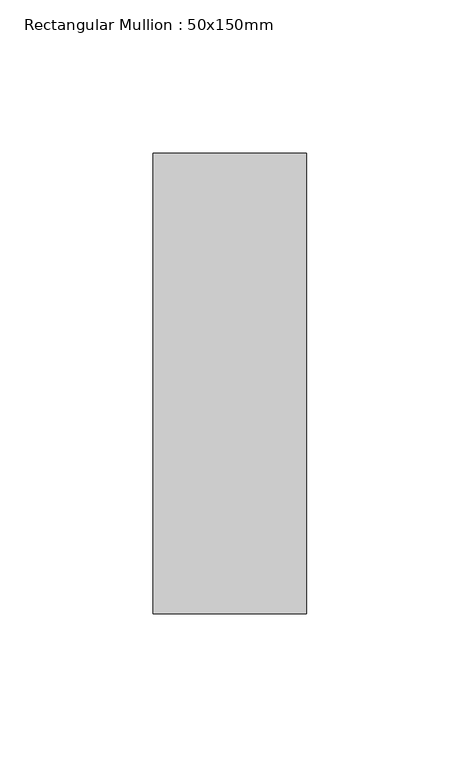
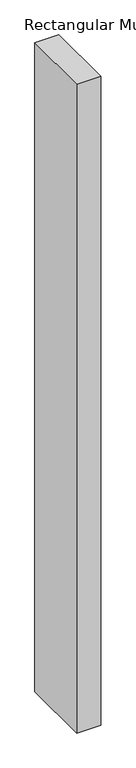
"""IFC4 building model written with IfcOpenShell, lengths in millimetres: member geometry, Rectangular Mullion : 50x150mm."""

import ifcopenshell
import ifcopenshell.guid

model = None  # the IFC model being written
_history = None  # IfcOwnerHistory: only IFC2X3 demands one
_inside = {}  # id of a spatial element -> (the spatial element, [elements in it])
_under = {}  # id of a project, library or spatial element -> (it, [spatial elements below it])
_declared = {}  # id of a project -> (the project, [libraries it declares])
_typed = {}  # id of a type object -> (the type object, [elements of that type])
_made_of = {}  # id of a material, layer set ... -> (it, [elements and type objects made of it])


def new_model(schema):
    """Start an empty IFC model of exactly this schema.

    Asked for "IFC4X3", IfcOpenShell would pick the latest addendum, in which some entities
    have other attributes; the version numbers below select the first issue.
    IFC2X3 requires an IfcOwnerHistory on every rooted entity: one is made here for all.
    """
    global model, _history
    if schema == "IFC4X3":
        model = ifcopenshell.file(schema_version=(4, 3, 0, 0))
    else:
        model = ifcopenshell.file(schema=schema)
    _inside.clear()
    _under.clear()
    _declared.clear()
    _typed.clear()
    _made_of.clear()
    _history = None
    if model.schema == "IFC2X3":
        org = make("IfcOrganization", Name="unknown")
        user = make(
            "IfcPersonAndOrganization",
            ThePerson=make("IfcPerson", FamilyName="unknown"),
            TheOrganization=org,
        )
        app = make(
            "IfcApplication",
            ApplicationDeveloper=org,
            Version="unknown",
            ApplicationFullName="unknown",
            ApplicationIdentifier="unknown",
        )
        _history = make(
            "IfcOwnerHistory",
            OwningUser=user,
            OwningApplication=app,
            ChangeAction="ADDED",
            CreationDate=0,
        )
    return model


def make(cls, **values):
    """One entity of the class cls with the attributes given. An attribute that is None is left unset."""
    return model.create_entity(
        cls, **{name: value for name, value in values.items() if value is not None}
    )


def rooted(cls, **values):
    """An entity with a GlobalId (a new one), such as an element, a storey or a relation."""
    return make(cls, GlobalId=ifcopenshell.guid.new(), OwnerHistory=_history, **values)


def si_unit(unit_type, name, prefix=None):
    """IfcSIUnit, for example si_unit("LENGTHUNIT", "METRE", prefix="MILLI")."""
    return make("IfcSIUnit", UnitType=unit_type, Prefix=prefix, Name=name)


def assignment(units):
    """IfcUnitAssignment: the units of a project."""
    return None if units is None else make("IfcUnitAssignment", Units=units)


def point(xyz):
    """IfcCartesianPoint."""
    return None if xyz is None else make("IfcCartesianPoint", Coordinates=xyz)


def direction(xyz):
    """IfcDirection."""
    return None if xyz is None else make("IfcDirection", DirectionRatios=xyz)


def frame(location, z_axis=None, x_axis=None):
    """IfcAxis2Placement3D, a coordinate frame: its origin and axes. An axis left out is left unset."""
    return make(
        "IfcAxis2Placement3D",
        Location=point(location),
        Axis=direction(z_axis),
        RefDirection=direction(x_axis),
    )


def origin():
    """The frame at (0, 0, 0) with its axes left unset."""
    return frame((0.0, 0.0, 0.0))


def place(relative_to, where):
    """IfcLocalPlacement: puts the frame where relative to a parent placement (None: the world)."""
    return make(
        "IfcLocalPlacement", PlacementRelTo=relative_to, RelativePlacement=where
    )


def context(
    kind, dimensions, precision=None, world=None, true_north=None, identifier=None
):
    """IfcGeometricRepresentationContext, for example the 3D "Model" context."""
    return make(
        "IfcGeometricRepresentationContext",
        ContextIdentifier=identifier,
        ContextType=kind,
        CoordinateSpaceDimension=dimensions,
        Precision=precision,
        WorldCoordinateSystem=world,
        TrueNorth=true_north,
    )


def project(units=None, contexts=None):
    """IfcProject with its units and contexts."""
    return rooted(
        "IfcProject",
        Name="project",
        RepresentationContexts=contexts,
        UnitsInContext=assignment(units),
    )


def spatial(cls, under=None, at=None, **own):
    """A site, building, storey or space (cls), placed at a placement, below another one or the project."""
    s = rooted(cls, ObjectPlacement=at, **own)
    if under is not None:
        _under.setdefault(under.id(), (under, []))[1].append(s)
    return s


def polyline(points):
    """IfcPolyline through the points."""
    return make("IfcPolyline", Points=[point(p) for p in points])


def outline(outer, holes=None, kind="AREA"):
    """IfcArbitraryClosedProfileDef: a profile drawn as a closed curve; with holes, ...WithVoids."""
    if holes is None:
        return make("IfcArbitraryClosedProfileDef", ProfileType=kind, OuterCurve=outer)
    return make(
        "IfcArbitraryProfileDefWithVoids",
        ProfileType=kind,
        OuterCurve=outer,
        InnerCurves=holes,
    )


def extrude(swept, where, along, depth):
    """IfcExtrudedAreaSolid: the profile swept, set in the frame where, extruded along a direction by depth."""
    return make(
        "IfcExtrudedAreaSolid",
        SweptArea=swept,
        Position=where,
        ExtrudedDirection=direction(along),
        Depth=depth,
    )


def shape(context_of_items, identifier, shape_type, items):
    """IfcShapeRepresentation: the items that make up one representation, for example the "Body"."""
    return make(
        "IfcShapeRepresentation",
        ContextOfItems=context_of_items,
        RepresentationIdentifier=identifier,
        RepresentationType=shape_type,
        Items=items,
    )


def source(mapping_origin, context_of_items, identifier, shape_type, items):
    """IfcRepresentationMap: a shape defined once, which mapped items show again and again."""
    return make(
        "IfcRepresentationMap",
        MappingOrigin=mapping_origin,
        MappedRepresentation=shape(context_of_items, identifier, shape_type, items),
    )


def transform(
    local_origin,
    x_axis=None,
    y_axis=None,
    z_axis=None,
    scale=None,
    scale2=None,
    scale3=None,
    uniform=True,
):
    """IfcCartesianTransformationOperator3D, or its non-uniform kind. x_axis, y_axis, z_axis: its Axis1, 2, 3."""
    if uniform:
        return make(
            "IfcCartesianTransformationOperator3D",
            Axis1=direction(x_axis),
            Axis2=direction(y_axis),
            LocalOrigin=point(local_origin),
            Scale=scale,
            Axis3=direction(z_axis),
        )
    return make(
        "IfcCartesianTransformationOperator3DnonUniform",
        Axis1=direction(x_axis),
        Axis2=direction(y_axis),
        LocalOrigin=point(local_origin),
        Scale=scale,
        Axis3=direction(z_axis),
        Scale2=scale2,
        Scale3=scale3,
    )


def mapped(mapping_source, mapping_target):
    """IfcMappedItem: shows the shape of a source again, moved by a transform."""
    return make(
        "IfcMappedItem", MappingSource=mapping_source, MappingTarget=mapping_target
    )


def made_of(thing, what):
    """Note that an element or type object is made of a material, layer set ...; save() writes the relation."""
    if what is not None:
        _made_of.setdefault(what.id(), (what, []))[1].append(thing)
    return thing


def element(
    cls,
    number,
    at=None,
    inside=None,
    cuts=None,
    type_object=None,
    material=None,
    context=None,
    identifier="Body",
    shape_type=None,
    held_by="IfcProductDefinitionShape",
    body=None,
    shapes=None,
    **own,
):
    """One element of the class cls, such as IfcWall. Its Tag is "e" and its number.

    at: its placement. inside: the storey or other place that contains it. cuts: it is an
    opening in that element (IfcRelVoidsElement). A single representation is given by context,
    identifier, shape_type and body (its items); several are given by shapes. held_by: the class
    of the entity that holds the representations. save() writes the other relations.
    """
    e = rooted(cls, Tag="e%d" % number, ObjectPlacement=at, **own)
    if body is not None:
        shapes = [shape(context, identifier, shape_type, body)]
    if shapes is not None:
        e.Representation = make(held_by, Representations=shapes)
    if inside is not None:
        _inside.setdefault(inside.id(), (inside, []))[1].append(e)
    if cuts is not None:
        rooted(
            "IfcRelVoidsElement", RelatingBuildingElement=cuts, RelatedOpeningElement=e
        )
    if type_object is not None:
        _typed.setdefault(type_object.id(), (type_object, []))[1].append(e)
    return made_of(e, material)


def aggregate(whole, parts):
    """IfcRelAggregates: a whole, such as a stair, and the parts it consists of."""
    return rooted("IfcRelAggregates", RelatingObject=whole, RelatedObjects=parts)


def save(model, path):
    """Write the relations noted so far, then the file.

    IfcRelAggregates (storeys below a building ...), IfcRelContainedInSpatialStructure (elements
    in a storey), IfcRelDefinesByType, IfcRelAssociatesMaterial and IfcRelDeclares: one each for
    every whole, place, type object, material and project.
    """
    for whole, parts in _under.values():
        aggregate(whole, parts)
    for where, things in _inside.values():
        rooted(
            "IfcRelContainedInSpatialStructure",
            RelatedElements=things,
            RelatingStructure=where,
        )
    for kind, things in _typed.values():
        rooted("IfcRelDefinesByType", RelatedObjects=things, RelatingType=kind)
    for what, things in _made_of.values():
        rooted("IfcRelAssociatesMaterial", RelatedObjects=things, RelatingMaterial=what)
    for by, libraries in _declared.values():
        rooted("IfcRelDeclares", RelatingContext=by, RelatedDefinitions=libraries)
    model.write(path)


def rectangular_mullion_50x150mm_2a0b7483(model_context):
    return source(origin(), model_context, "Body", "SweptSolid", [
        extrude(outline(polyline([(0.0, 75.0), (0.0, -75.0), (-50.0, -75.0), (-50.0, 75.0), (0.0, 75.0)])), frame((0.0, 0.0, -1425.0000002), z_axis=(0.0, 0.0, 1.0), x_axis=(1.0, 0.0, 0.0)), (0.0, 0.0, 1.0), 1425.0000002),
    ])


if __name__ == "__main__":
    model = new_model("IFC4")
    model_context = context("Model", 3, world=origin())
    ifc_project = project(units=[si_unit("LENGTHUNIT", "METRE", prefix="MILLI")], contexts=[model_context])
    site = spatial("IfcSite", under=ifc_project)
    building = spatial("IfcBuilding", under=site)
    placement = place(None, origin())
    rectangular_mullion_50x150mm_shape = rectangular_mullion_50x150mm_2a0b7483(model_context)
    element("IfcMember", 1, ObjectType="Rectangular Mullion : 50x150mm", at=placement, inside=building, context=model_context, shape_type="MappedRepresentation", body=[
        mapped(rectangular_mullion_50x150mm_shape, transform((0.0, 0.0, 0.0), x_axis=(1.0, 0.0, 0.0), y_axis=(0.0, 1.0, 0.0), z_axis=(0.0, 0.0, 1.0))),
    ])
    save(model, "model.ifc")

# Revit data of these elements
# Type "Rectangular Mullion : 50x150mm"
#   Keynote = "H11"
#   built-in parameter 1007304 = 0.492126 (stored number, unit not read)
#   built-in parameter 1007301 = 0.082021 (stored number, unit not read)
#   built-in parameter 1007300 = 0.082021 (stored number, unit not read)
# Element 1 (IfcMember, "Rectangular Mullion : 50x150mm")
#   Materials on its faces: "Aluminium"
# Materials
#   "Aluminium": class "Metal", colour RGB 247 247 247, transparency 0, Description = "Aluminium 6061", Cost = 0
